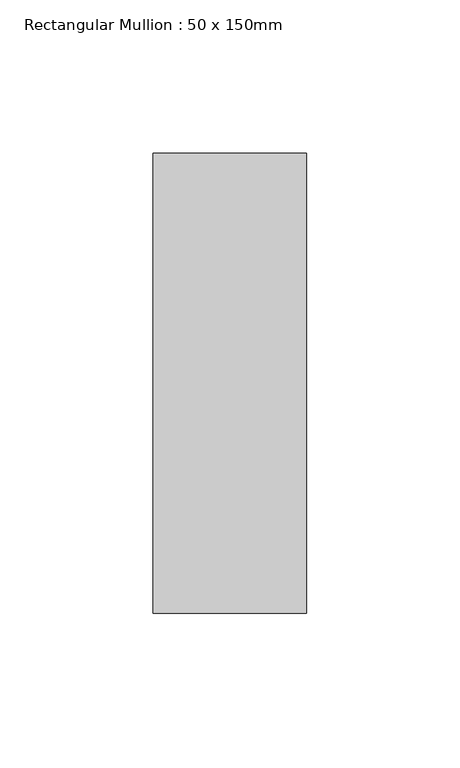
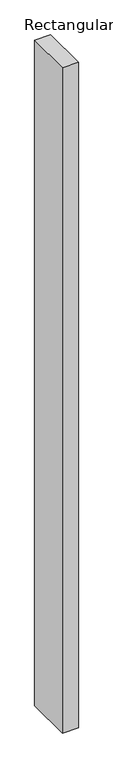
"""IFC4 building model written with IfcOpenShell, lengths in millimetres: member geometry, Rectangular Mullion : 50 x 150mm."""

from ifc_helpers import new_model, si_unit, frame, origin, place, context, project, spatial, polyline, outline, extrude, source, transform, mapped, element, save


def rectangular_mullion_50_x_150mm_9cef7b28(model_context):
    return source(origin(), model_context, "Body", "SweptSolid", [
        extrude(outline(polyline([(25.0, 75.0), (25.0, -75.0), (-25.0, -75.0), (-25.0, 75.0), (25.0, 75.0)])), frame((0.0, 0.0, -2200.0), z_axis=(0.0, 0.0, 1.0), x_axis=(1.0, 0.0, 0.0)), (0.0, 0.0, 1.0), 2200.0),
    ])


if __name__ == "__main__":
    model = new_model("IFC4")
    model_context = context("Model", 3, world=origin())
    ifc_project = project(units=[si_unit("LENGTHUNIT", "METRE", prefix="MILLI")], contexts=[model_context])
    site = spatial("IfcSite", under=ifc_project)
    building = spatial("IfcBuilding", under=site)
    placement = place(None, origin())
    rectangular_mullion_50_x_150mm_shape = rectangular_mullion_50_x_150mm_9cef7b28(model_context)
    element("IfcMember", 1, ObjectType="Rectangular Mullion : 50 x 150mm", at=placement, inside=building, context=model_context, shape_type="MappedRepresentation", body=[
        mapped(rectangular_mullion_50_x_150mm_shape, transform((0.0, 0.0, 0.0), x_axis=(1.0, 0.0, 0.0), y_axis=(0.0, 1.0, 0.0), z_axis=(0.0, 0.0, 1.0))),
    ])
    save(model, "model.ifc")

# Revit data of these elements
# Type "Rectangular Mullion : 50 x 150mm"
#   Keynote = "H11"
#   built-in parameter 1007304 = 0.492126 (stored number, unit not read)
#   built-in parameter 1007301 = 0.082021 (stored number, unit not read)
#   built-in parameter 1007300 = 0.082021 (stored number, unit not read)
# Element 1 (IfcMember, "Rectangular Mullion : 50 x 150mm")
#   Materials on its faces: "Aluminium"
# Materials
#   "Aluminium": class "Metal", colour RGB 247 247 247, transparency 0, Description = "Aluminium 6061", Cost = 0
